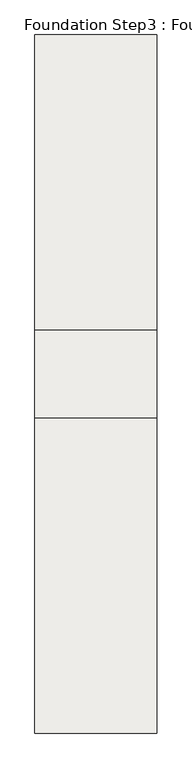
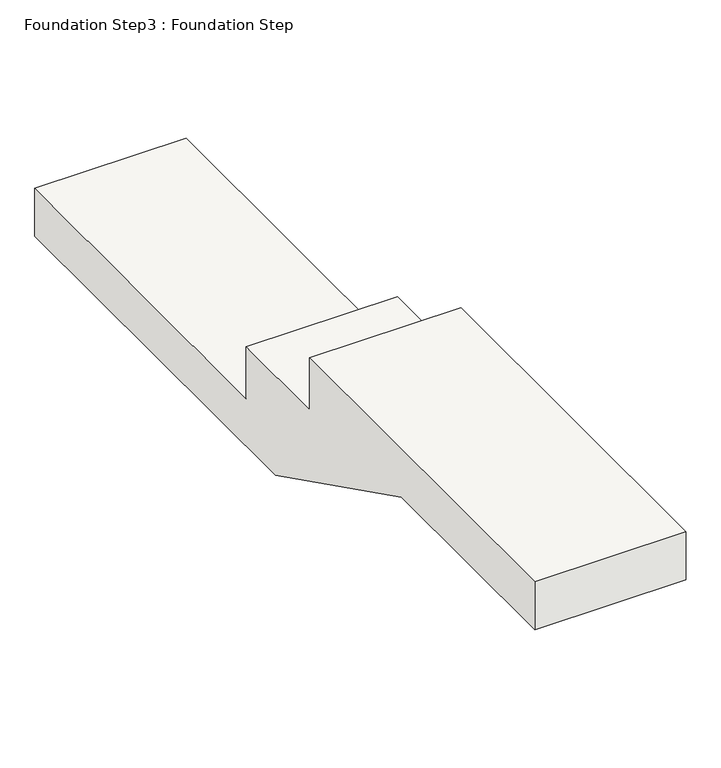
"""IFC4 building model written with IfcOpenShell, lengths in millimetres: slab geometry, Foundation Step3 : Foundation Step."""

from ifc_helpers import new_model, si_unit, frame, origin, place, context, project, spatial, polyline, outline, extrude, source, transform, mapped, element, save


def foundation_step3_foundation_step_6bcc790d(model_context):
    return source(origin(), model_context, "Body", "SweptSolid", [
        extrude(outline(polyline([(10612.1768471, -1092.2), (10612.1768471, -1422.4), (11272.5768471, -1422.4), (11272.5768471, -1752.6), (13485.5518471, -1752.6), (13485.5518471, -2057.4), (10967.7768471, -2057.4), (9646.9768471, -1397.0), (8253.7505048, -1397.0), (8253.7505048, -1092.2), (10612.1768471, -1092.2)])), frame((-45451.7600821, 0.0, 0.0), z_axis=(1.0, 0.0, 0.0), x_axis=(0.0, 1.0, 0.0)), (0.0, 0.0, 1.0), 914.4),
    ])


if __name__ == "__main__":
    model = new_model("IFC4")
    model_context = context("Model", 3, world=origin())
    ifc_project = project(units=[si_unit("LENGTHUNIT", "METRE", prefix="MILLI")], contexts=[model_context])
    site = spatial("IfcSite", under=ifc_project)
    building = spatial("IfcBuilding", under=site)
    placement = place(None, origin())
    foundation_step3_foundation_step_shape = foundation_step3_foundation_step_6bcc790d(model_context)
    element("IfcSlab", 1, ObjectType="Foundation Step3 : Foundation Step", at=placement, inside=building, context=model_context, shape_type="MappedRepresentation", body=[
        mapped(foundation_step3_foundation_step_shape, transform((0.0, 0.0, 0.0), x_axis=(1.0, 0.0, 0.0), y_axis=(0.0, 1.0, 0.0), z_axis=(0.0, 0.0, 1.0))),
    ])
    save(model, "model.ifc")

# Revit data of these elements
# Type "Foundation Step3 : Foundation Step"
#   Structural Material = Concrete, Cast-in-Place gray
# Materials
#   "Concrete, Cast-in-Place gray": class "Concrete", colour RGB 192 192 192, transparency 0, Description = "Cast-in-place concrete", Cost = 0
